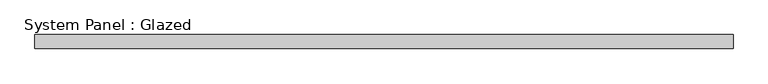
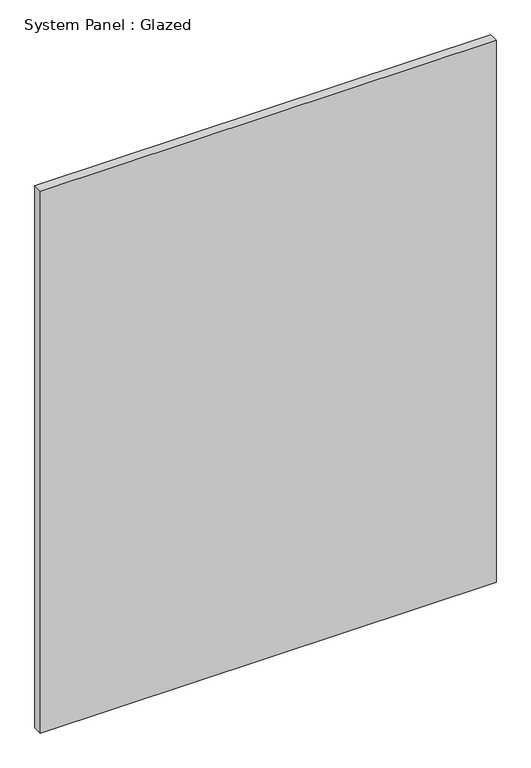
"""IFC4 building model written with IfcOpenShell, lengths in millimetres: plate geometry, System Panel : Glazed."""

from ifc_helpers import new_model, si_unit, origin, origin_with_axes, place, context, project, spatial, polyline, outline, extrude, source, transform, mapped, element, save


def system_panel_glazed_d4804bae(model_context):
    return source(origin(), model_context, "Body", "SweptSolid", [
        extrude(outline(polyline([(620.5541356, 24.5), (-620.5541356, 24.5), (-620.5541356, 49.5), (620.5541356, 49.5), (620.5541356, 24.5)])), origin_with_axes(), (0.0, 0.0, 1.0), 1560.0991456),
    ])


if __name__ == "__main__":
    model = new_model("IFC4")
    model_context = context("Model", 3, world=origin())
    ifc_project = project(units=[si_unit("LENGTHUNIT", "METRE", prefix="MILLI")], contexts=[model_context])
    site = spatial("IfcSite", under=ifc_project)
    building = spatial("IfcBuilding", under=site)
    placement = place(None, origin())
    system_panel_glazed_shape = system_panel_glazed_d4804bae(model_context)
    element("IfcPlate", 1, ObjectType="System Panel : Glazed", at=placement, inside=building, context=model_context, shape_type="MappedRepresentation", body=[
        mapped(system_panel_glazed_shape, transform((0.0, 0.0, 0.0), x_axis=(1.0, 0.0, 0.0), y_axis=(0.0, 1.0, 0.0), z_axis=(0.0, 0.0, 1.0))),
    ])
    save(model, "model.ifc")

# Revit data of these elements
# Type "System Panel : Glazed"
#   Construction Type Id = "GSP4R"
#   Analytic Construction = "1/8 in Pilkington single glazing"
#   Visual Light Transmittance = 0.9
#   Solar Heat Gain Coefficient = 0.86
#   Heat Transfer Coefficient (U) = 6.7069 W/(m²·K)
#   Define Thermal Properties by = 1
# Element 1 (IfcPlate, "System Panel : Glazed")
#   Materials on its faces: "Glass"
# Materials
#   "Glass": class "Glass", colour RGB 0 128 192, transparency 0.9, Description = "Soda Lime Glass", Cost = 0
